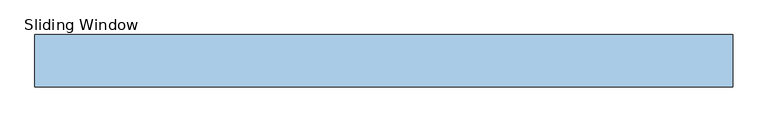
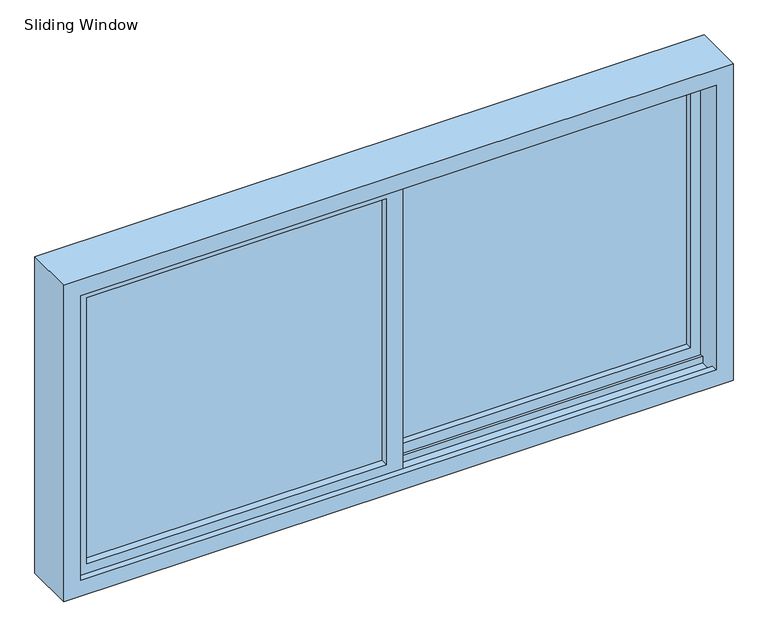
"""IFC4 building model written with IfcOpenShell, lengths in millimetres: window geometry, Sliding Window : H_WD_AR_B11_Sliding_Steel Window_DG_W2000xH1000."""

from ifc_helpers import new_model, si_unit, frame, origin, place, context, project, spatial, polyline, outline, extrude, faceted_brep, source, transform, mapped, element, save


def sliding_window_5e64f0fd(model_context):
    return source(origin(), model_context, "Body", "SolidModel", [
        extrude(outline(polyline([(920.0, 27.5), (25.0, 27.5), (25.0, 32.5), (920.0, 32.5), (920.0, 27.5)])), frame((0.0, 0.0, 680.0), z_axis=(0.0, 0.0, 1.0), x_axis=(1.0, 0.0, 0.0)), (0.0, 0.0, 1.0), 840.0),
        extrude(outline(polyline([(-25.0, -32.5), (-920.0, -32.5), (-920.0, -27.5), (-25.0, -27.5), (-25.0, -32.5)])), frame((0.0, 0.0, 680.0), z_axis=(0.0, 0.0, 1.0), x_axis=(1.0, 0.0, 0.0)), (0.0, 0.0, 1.0), 840.0),
        extrude(outline(polyline([(630.0, -970.0), (630.0, 25.0), (1570.0, 25.0), (1570.0, -970.0), (630.0, -970.0)]), holes=[polyline([(1520.0, -920.0), (1520.0, -25.0), (680.0, -25.0), (680.0, -920.0), (1520.0, -920.0)])]), frame((0.0, -55.0, 0.0), z_axis=(0.0, 1.0, 0.0), x_axis=(0.0, 0.0, 1.0)), (0.0, 0.0, 1.0), 47.5),
        extrude(outline(polyline([(630.0, -25.0), (630.0, 970.0), (1570.0, 970.0), (1570.0, -25.0), (630.0, -25.0)]), holes=[polyline([(1520.0, 25.0), (1520.0, 920.0), (680.0, 920.0), (680.0, 25.0), (1520.0, 25.0)])]), frame((0.0, 7.5, 0.0), z_axis=(0.0, 1.0, 0.0), x_axis=(0.0, 0.0, 1.0)), (0.0, 0.0, 1.0), 45.0),
        faceted_brep([(-1000.0, 75.0, 1600.0), (-1000.0, 75.0, 600.0), (-1000.0, -75.0, 600.0), (-1000.0, -75.0, 1600.0), (1000.0, 75.0, 1600.0), (1000.0, 75.0, 600.0), (950.0, 75.0, 650.0), (950.0, 75.0, 1550.0), (-950.0, 75.0, 1550.0), (-950.0, 75.0, 650.0), (1000.0, -75.0, 600.0), (1000.0, -75.0, 1600.0), (-950.0, -75.0, 1550.0), (950.0, -75.0, 1550.0), (950.0, -75.0, 650.0), (-950.0, -75.0, 650.0), (950.0, 55.0, 650.0), (950.0, 55.0, 1550.0), (-950.0, 55.0, 1550.0), (-950.0, 55.0, 1570.0), (-950.0, 5.0, 1570.0), (-950.0, 5.0, 1550.0), (-950.0, -5.0, 1550.0), (-950.0, -5.0, 650.0), (-950.0, 5.0, 650.0), (-950.0, 5.0, 630.0), (-950.0, 55.0, 630.0), (-950.0, 55.0, 650.0), (950.0, -5.0, 650.0), (950.0, 5.0, 650.0), (950.0, -5.0, 630.0), (950.0, -55.0, 630.0), (950.0, -55.0, 650.0), (950.0, -55.0, 1550.0), (950.0, -55.0, 1570.0), (950.0, -5.0, 1570.0), (950.0, -5.0, 1550.0), (950.0, 5.0, 1550.0), (970.0, 5.0, 1570.0), (970.0, 5.0, 630.0), (-970.0, -5.0, 1570.0), (-970.0, -5.0, 630.0), (970.0, 55.0, 1570.0), (970.0, 55.0, 630.0), (-970.0, -55.0, 630.0), (-950.0, -55.0, 1550.0), (-950.0, -55.0, 650.0), (-970.0, -55.0, 1570.0)], [[[0, 1, 2, 3]], [[4, 5, 1, 0], [6, 7, 8, 9]], [[1, 5, 10, 2]], [[10, 11, 3, 2], [12, 13, 14, 15]], [[7, 6, 16, 17]], [[9, 8, 18, 19, 20, 21, 22, 23, 24, 25, 26, 27]], [[16, 6, 9, 27]], [[5, 4, 11, 10]], [[28, 29, 24, 23]], [[28, 30, 31, 32, 14, 13, 33, 34, 35, 36, 37, 29]], [[29, 37, 21, 20, 38, 39, 25, 24]], [[40, 41, 30, 28, 23, 22, 36, 35]], [[39, 38, 42, 43]], [[39, 43, 26, 25]], [[43, 42, 19, 18, 17, 16, 27, 26]], [[41, 44, 31, 30]], [[45, 46, 32, 31, 44, 47, 34, 33]], [[46, 15, 14, 32]], [[12, 15, 46, 45]], [[47, 44, 41, 40]], [[3, 11, 4, 0]], [[7, 17, 18, 8]], [[37, 36, 22, 21]], [[42, 38, 20, 19]], [[12, 45, 33, 13]], [[47, 40, 35, 34]]]),
    ])


if __name__ == "__main__":
    model = new_model("IFC4")
    model_context = context("Model", 3, world=origin())
    ifc_project = project(units=[si_unit("LENGTHUNIT", "METRE", prefix="MILLI")], contexts=[model_context])
    site = spatial("IfcSite", under=ifc_project)
    building = spatial("IfcBuilding", under=site)
    placement = place(None, origin())
    sliding_window_shape = sliding_window_5e64f0fd(model_context)
    element("IfcWindow", 1, ObjectType="Sliding Window : H_WD_AR_B11_Sliding_Steel Window_DG_W2000xH1000", at=placement, inside=building, context=model_context, shape_type="MappedRepresentation", body=[
        mapped(sliding_window_shape, transform((0.0, 0.0, 0.0), x_axis=(1.0, 0.0, 0.0), y_axis=(0.0, 1.0, 0.0), z_axis=(0.0, 0.0, 1.0))),
    ])
    save(model, "model.ifc")

# Revit data of these elements
# Type "Sliding Window : H_WD_AR_B11_Sliding_Steel Window_DG_W2000xH1000"
#   Description = "Steel Frame + 2 x T=6mm + T12mm Air Space"
#   Type Mark = ""
#   Analytic Construction = "<None>"
#   창 두께 = 150 mm
#   Visual Light Transmittance = 0.88
#   Thermal Resistance (R) = 0.271106 (m²·K)/W
#   Solar Heat Gain Coefficient = 0.81
#   Height = 1000 mm
#   Heat Transfer Coefficient (U) = 6.2426 W/(m²·K)
#   기본 씰 높이 = 600 mm
#   Width = 2000 mm
#   Define Thermal Properties by = 1
#   창 패널 = none
#   창 프레임 = none
#   Construction Type Id = ""
#   Wall Closure = (empty or 0)
